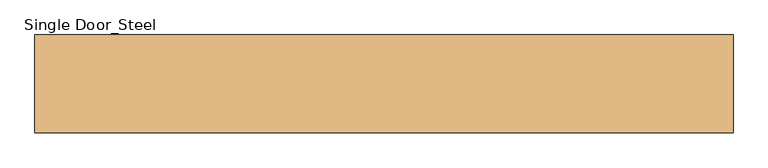
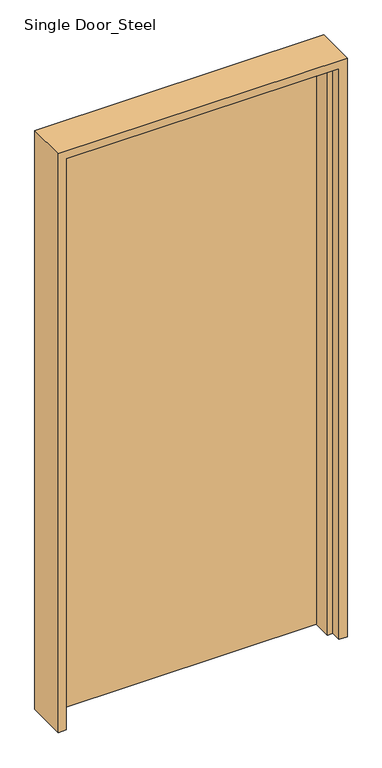
"""IFC4 building model written with IfcOpenShell, lengths in millimetres: door geometry, Single Door_Steel : H_DR_AR B12_Door_Single_W1100xH2280_FR 1.0H_FSD-1."""

import ifcopenshell
import ifcopenshell.guid

model = None  # the IFC model being written
_history = None  # IfcOwnerHistory: only IFC2X3 demands one
_inside = {}  # id of a spatial element -> (the spatial element, [elements in it])
_under = {}  # id of a project, library or spatial element -> (it, [spatial elements below it])
_declared = {}  # id of a project -> (the project, [libraries it declares])
_typed = {}  # id of a type object -> (the type object, [elements of that type])
_made_of = {}  # id of a material, layer set ... -> (it, [elements and type objects made of it])


def new_model(schema):
    """Start an empty IFC model of exactly this schema.

    Asked for "IFC4X3", IfcOpenShell would pick the latest addendum, in which some entities
    have other attributes; the version numbers below select the first issue.
    IFC2X3 requires an IfcOwnerHistory on every rooted entity: one is made here for all.
    """
    global model, _history
    if schema == "IFC4X3":
        model = ifcopenshell.file(schema_version=(4, 3, 0, 0))
    else:
        model = ifcopenshell.file(schema=schema)
    _inside.clear()
    _under.clear()
    _declared.clear()
    _typed.clear()
    _made_of.clear()
    _history = None
    if model.schema == "IFC2X3":
        org = make("IfcOrganization", Name="unknown")
        user = make(
            "IfcPersonAndOrganization",
            ThePerson=make("IfcPerson", FamilyName="unknown"),
            TheOrganization=org,
        )
        app = make(
            "IfcApplication",
            ApplicationDeveloper=org,
            Version="unknown",
            ApplicationFullName="unknown",
            ApplicationIdentifier="unknown",
        )
        _history = make(
            "IfcOwnerHistory",
            OwningUser=user,
            OwningApplication=app,
            ChangeAction="ADDED",
            CreationDate=0,
        )
    return model


def make(cls, **values):
    """One entity of the class cls with the attributes given. An attribute that is None is left unset."""
    return model.create_entity(
        cls, **{name: value for name, value in values.items() if value is not None}
    )


def rooted(cls, **values):
    """An entity with a GlobalId (a new one), such as an element, a storey or a relation."""
    return make(cls, GlobalId=ifcopenshell.guid.new(), OwnerHistory=_history, **values)


def si_unit(unit_type, name, prefix=None):
    """IfcSIUnit, for example si_unit("LENGTHUNIT", "METRE", prefix="MILLI")."""
    return make("IfcSIUnit", UnitType=unit_type, Prefix=prefix, Name=name)


def assignment(units):
    """IfcUnitAssignment: the units of a project."""
    return None if units is None else make("IfcUnitAssignment", Units=units)


def point(xyz):
    """IfcCartesianPoint."""
    return None if xyz is None else make("IfcCartesianPoint", Coordinates=xyz)


def direction(xyz):
    """IfcDirection."""
    return None if xyz is None else make("IfcDirection", DirectionRatios=xyz)


def frame(location, z_axis=None, x_axis=None):
    """IfcAxis2Placement3D, a coordinate frame: its origin and axes. An axis left out is left unset."""
    return make(
        "IfcAxis2Placement3D",
        Location=point(location),
        Axis=direction(z_axis),
        RefDirection=direction(x_axis),
    )


def origin():
    """The frame at (0, 0, 0) with its axes left unset."""
    return frame((0.0, 0.0, 0.0))


def origin_with_axes():
    """The frame at (0, 0, 0) with the z axis (0, 0, 1) and the x axis (1, 0, 0) written out."""
    return frame((0.0, 0.0, 0.0), z_axis=(0.0, 0.0, 1.0), x_axis=(1.0, 0.0, 0.0))


def place(relative_to, where):
    """IfcLocalPlacement: puts the frame where relative to a parent placement (None: the world)."""
    return make(
        "IfcLocalPlacement", PlacementRelTo=relative_to, RelativePlacement=where
    )


def context(
    kind, dimensions, precision=None, world=None, true_north=None, identifier=None
):
    """IfcGeometricRepresentationContext, for example the 3D "Model" context."""
    return make(
        "IfcGeometricRepresentationContext",
        ContextIdentifier=identifier,
        ContextType=kind,
        CoordinateSpaceDimension=dimensions,
        Precision=precision,
        WorldCoordinateSystem=world,
        TrueNorth=true_north,
    )


def project(units=None, contexts=None):
    """IfcProject with its units and contexts."""
    return rooted(
        "IfcProject",
        Name="project",
        RepresentationContexts=contexts,
        UnitsInContext=assignment(units),
    )


def spatial(cls, under=None, at=None, **own):
    """A site, building, storey or space (cls), placed at a placement, below another one or the project."""
    s = rooted(cls, ObjectPlacement=at, **own)
    if under is not None:
        _under.setdefault(under.id(), (under, []))[1].append(s)
    return s


def polyline(points):
    """IfcPolyline through the points."""
    return make("IfcPolyline", Points=[point(p) for p in points])


def outline(outer, holes=None, kind="AREA"):
    """IfcArbitraryClosedProfileDef: a profile drawn as a closed curve; with holes, ...WithVoids."""
    if holes is None:
        return make("IfcArbitraryClosedProfileDef", ProfileType=kind, OuterCurve=outer)
    return make(
        "IfcArbitraryProfileDefWithVoids",
        ProfileType=kind,
        OuterCurve=outer,
        InnerCurves=holes,
    )


def extrude(swept, where, along, depth):
    """IfcExtrudedAreaSolid: the profile swept, set in the frame where, extruded along a direction by depth."""
    return make(
        "IfcExtrudedAreaSolid",
        SweptArea=swept,
        Position=where,
        ExtrudedDirection=direction(along),
        Depth=depth,
    )


def faces_of(points, faces, orient=None, outer=None):
    """IfcFace entities. A face is a list of loops; a loop is a list of indices into points, from 0.

    orient and outer hold one flag for each loop. By default every Orientation is true, the
    first loop of a face is its IfcFaceOuterBound and the others are IfcFaceBound.
    """
    made = []
    for i, loops in enumerate(faces):
        bounds = []
        for j, loop in enumerate(loops):
            is_outer = j == 0 if outer is None else outer[i][j]
            bounds.append(
                make(
                    "IfcFaceOuterBound" if is_outer else "IfcFaceBound",
                    Bound=make("IfcPolyLoop", Polygon=[points[k] for k in loop]),
                    Orientation=True if orient is None else orient[i][j],
                )
            )
        made.append(make("IfcFace", Bounds=bounds))
    return made


def faceted_brep(points, faces, orient=None, outer=None, voids=None):
    """IfcFacetedBrep: a solid bounded by flat faces; with voids (closed shells), ...WithVoids."""
    shared = [point(p) for p in points]
    hull = make("IfcClosedShell", CfsFaces=faces_of(shared, faces, orient, outer))
    if voids is None:
        return make("IfcFacetedBrep", Outer=hull)
    return make(
        "IfcFacetedBrepWithVoids",
        Outer=hull,
        Voids=[
            make(cls, CfsFaces=faces_of(shared, fs, o, b)) for cls, fs, o, b in voids
        ],
    )


def shape(context_of_items, identifier, shape_type, items):
    """IfcShapeRepresentation: the items that make up one representation, for example the "Body"."""
    return make(
        "IfcShapeRepresentation",
        ContextOfItems=context_of_items,
        RepresentationIdentifier=identifier,
        RepresentationType=shape_type,
        Items=items,
    )


def source(mapping_origin, context_of_items, identifier, shape_type, items):
    """IfcRepresentationMap: a shape defined once, which mapped items show again and again."""
    return make(
        "IfcRepresentationMap",
        MappingOrigin=mapping_origin,
        MappedRepresentation=shape(context_of_items, identifier, shape_type, items),
    )


def transform(
    local_origin,
    x_axis=None,
    y_axis=None,
    z_axis=None,
    scale=None,
    scale2=None,
    scale3=None,
    uniform=True,
):
    """IfcCartesianTransformationOperator3D, or its non-uniform kind. x_axis, y_axis, z_axis: its Axis1, 2, 3."""
    if uniform:
        return make(
            "IfcCartesianTransformationOperator3D",
            Axis1=direction(x_axis),
            Axis2=direction(y_axis),
            LocalOrigin=point(local_origin),
            Scale=scale,
            Axis3=direction(z_axis),
        )
    return make(
        "IfcCartesianTransformationOperator3DnonUniform",
        Axis1=direction(x_axis),
        Axis2=direction(y_axis),
        LocalOrigin=point(local_origin),
        Scale=scale,
        Axis3=direction(z_axis),
        Scale2=scale2,
        Scale3=scale3,
    )


def mapped(mapping_source, mapping_target):
    """IfcMappedItem: shows the shape of a source again, moved by a transform."""
    return make(
        "IfcMappedItem", MappingSource=mapping_source, MappingTarget=mapping_target
    )


def made_of(thing, what):
    """Note that an element or type object is made of a material, layer set ...; save() writes the relation."""
    if what is not None:
        _made_of.setdefault(what.id(), (what, []))[1].append(thing)
    return thing


def element(
    cls,
    number,
    at=None,
    inside=None,
    cuts=None,
    type_object=None,
    material=None,
    context=None,
    identifier="Body",
    shape_type=None,
    held_by="IfcProductDefinitionShape",
    body=None,
    shapes=None,
    **own,
):
    """One element of the class cls, such as IfcWall. Its Tag is "e" and its number.

    at: its placement. inside: the storey or other place that contains it. cuts: it is an
    opening in that element (IfcRelVoidsElement). A single representation is given by context,
    identifier, shape_type and body (its items); several are given by shapes. held_by: the class
    of the entity that holds the representations. save() writes the other relations.
    """
    e = rooted(cls, Tag="e%d" % number, ObjectPlacement=at, **own)
    if body is not None:
        shapes = [shape(context, identifier, shape_type, body)]
    if shapes is not None:
        e.Representation = make(held_by, Representations=shapes)
    if inside is not None:
        _inside.setdefault(inside.id(), (inside, []))[1].append(e)
    if cuts is not None:
        rooted(
            "IfcRelVoidsElement", RelatingBuildingElement=cuts, RelatedOpeningElement=e
        )
    if type_object is not None:
        _typed.setdefault(type_object.id(), (type_object, []))[1].append(e)
    return made_of(e, material)


def aggregate(whole, parts):
    """IfcRelAggregates: a whole, such as a stair, and the parts it consists of."""
    return rooted("IfcRelAggregates", RelatingObject=whole, RelatedObjects=parts)


def save(model, path):
    """Write the relations noted so far, then the file.

    IfcRelAggregates (storeys below a building ...), IfcRelContainedInSpatialStructure (elements
    in a storey), IfcRelDefinesByType, IfcRelAssociatesMaterial and IfcRelDeclares: one each for
    every whole, place, type object, material and project.
    """
    for whole, parts in _under.values():
        aggregate(whole, parts)
    for where, things in _inside.values():
        rooted(
            "IfcRelContainedInSpatialStructure",
            RelatedElements=things,
            RelatingStructure=where,
        )
    for kind, things in _typed.values():
        rooted("IfcRelDefinesByType", RelatedObjects=things, RelatingType=kind)
    for what, things in _made_of.values():
        rooted("IfcRelAssociatesMaterial", RelatedObjects=things, RelatingMaterial=what)
    for by, libraries in _declared.values():
        rooted("IfcRelDeclares", RelatingContext=by, RelatedDefinitions=libraries)
    model.write(path)


def single_door_steel_2a7c0b4f(model_context):
    return source(origin(), model_context, "Body", "SolidModel", [
        extrude(outline(polyline([(505.0, 75.0), (505.0, 35.0), (-505.0, 35.0), (-505.0, 75.0), (505.0, 75.0)])), origin_with_axes(), (0.0, 0.0, 1.0), 2235.0),
        faceted_brep([(505.0, 75.0, 0.0), (535.0, 75.0, 0.0), (535.0, -75.0, 0.0), (505.0, -75.0, 0.0), (505.0, -35.0, 0.0), (485.0, -35.0, 0.0), (485.0, 35.0, 0.0), (505.0, 35.0, 0.0), (-505.0, 75.0, 0.0), (-505.0, 35.0, 0.0), (-485.0, 35.0, 0.0), (-485.0, -35.0, 0.0), (-505.0, -35.0, 0.0), (-505.0, -75.0, 0.0), (-535.0, -75.0, 0.0), (-535.0, 75.0, 0.0), (505.0, 75.0, 2235.0), (-505.0, 75.0, 2235.0), (-535.0, 75.0, 2265.0), (535.0, 75.0, 2265.0), (535.0, -75.0, 2265.0), (-535.0, -75.0, 2265.0), (-505.0, -75.0, 2235.0), (505.0, -75.0, 2235.0), (505.0, -35.0, 2235.0), (-505.0, -35.0, 2235.0), (-485.0, -35.0, 2215.0), (485.0, -35.0, 2215.0), (485.0, 35.0, 2215.0), (-485.0, 35.0, 2215.0), (-505.0, 35.0, 2235.0), (505.0, 35.0, 2235.0)], [[[0, 1, 2, 3, 4, 5, 6, 7]], [[8, 9, 10, 11, 12, 13, 14, 15]], [[1, 0, 16, 17, 8, 15, 18, 19]], [[2, 1, 19, 20]], [[3, 2, 20, 21, 14, 13, 22, 23]], [[4, 3, 23, 24]], [[5, 4, 24, 25, 12, 11, 26, 27]], [[6, 5, 27, 28]], [[7, 6, 28, 29, 10, 9, 30, 31]], [[0, 7, 31, 16]], [[17, 30, 9, 8]], [[21, 18, 15, 14]], [[25, 22, 13, 12]], [[29, 26, 11, 10]], [[20, 19, 18, 21]], [[24, 23, 22, 25]], [[28, 27, 26, 29]], [[16, 31, 30, 17]]]),
    ])


if __name__ == "__main__":
    model = new_model("IFC4")
    model_context = context("Model", 3, world=origin())
    ifc_project = project(units=[si_unit("LENGTHUNIT", "METRE", prefix="MILLI")], contexts=[model_context])
    site = spatial("IfcSite", under=ifc_project)
    building = spatial("IfcBuilding", under=site)
    placement = place(None, origin())
    single_door_steel_shape = single_door_steel_2a7c0b4f(model_context)
    element("IfcDoor", 1, ObjectType="Single Door_Steel : H_DR_AR B12_Door_Single_W1100xH2280_FR 1.0H_FSD-1", at=placement, inside=building, context=model_context, shape_type="MappedRepresentation", body=[
        mapped(single_door_steel_shape, transform((0.0, 0.0, 0.0), x_axis=(1.0, 0.0, 0.0), y_axis=(0.0, 1.0, 0.0), z_axis=(0.0, 0.0, 1.0))),
    ])
    save(model, "model.ifc")

# Revit data of these elements
# Type "Single Door_Steel : H_DR_AR B12_Door_Single_W1100xH2280_FR 1.0H_FSD-1"
#   Type Mark = "441"
#   Analytic Construction = "<None>"
#   프레임 투영 외부. = 25 mm
#   프레임 투영 내부. = 25 mm
#   프레임 폭 = 75 mm
#   Height = 2280 mm
#   Width = 1100 mm
#   Define Thermal Properties by = 1
#   문 패널 = none
#   문 프레임 = none
#   Function = (empty or 0)
#   Wall Closure = (empty or 0)
